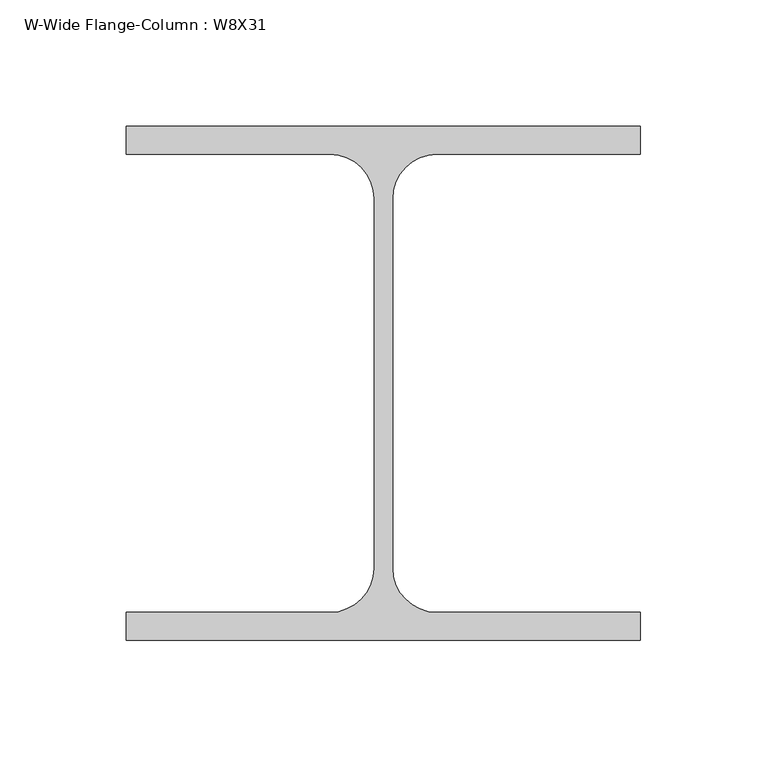
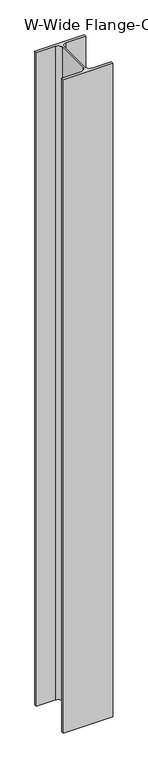
"""IFC4 building model written with IfcOpenShell, lengths in millimetres: column geometry, W-Wide Flange-Column : W8X31."""

from ifc_helpers import new_model, si_unit, point, frame_2d, origin, origin_with_axes, place, context, project, spatial, polyline, circle_curve, trimmed, segment, composite_curve, outline, extrude, source, transform, mapped, element, save


def w_wide_flange_column_w8x31_d6c08447(model_context):
    return source(origin(), model_context, "Body", "SweptSolid", [
        extrude(outline(composite_curve([segment(polyline([(101.6, 101.6), (101.6, 90.551), (21.1455, 90.551)]), True, "CONTINUOUS"), segment(trimmed(circle_curve(frame_2d((21.1455, 73.025)), 17.526), [point((21.1455, 90.551))], [point((3.6195, 73.025))], True, "CARTESIAN"), True, "CONTINUOUS"), segment(polyline([(3.6195, 73.025), (3.6195, -73.025)]), True, "CONTINUOUS"), segment(trimmed(circle_curve(frame_2d((21.1455, -73.025)), 17.526), [point((3.6195, -73.025))], [point((21.1455, -90.551))], True, "CARTESIAN"), True, "CONTINUOUS"), segment(polyline([(21.1455, -90.551), (101.6, -90.551), (101.6, -101.6), (-101.6, -101.6), (-101.6, -90.551), (-21.1455, -90.551)]), True, "CONTINUOUS"), segment(trimmed(circle_curve(frame_2d((-21.1455, -73.025)), 17.526), [point((-21.1455, -90.551))], [point((-3.6195, -73.025))], True, "CARTESIAN"), True, "CONTINUOUS"), segment(polyline([(-3.6195, -73.025), (-3.6195, 73.025)]), True, "CONTINUOUS"), segment(trimmed(circle_curve(frame_2d((-21.1455, 73.025)), 17.526), [point((-3.6195, 73.025))], [point((-21.1455, 90.551))], True, "CARTESIAN"), True, "CONTINUOUS"), segment(polyline([(-21.1455, 90.551), (-101.6, 90.551), (-101.6, 101.6), (101.6, 101.6)]), True, "CONTINUOUS")], self_intersect=False)), origin_with_axes(), (0.0, 0.0, 1.0), 2844.8),
    ])


if __name__ == "__main__":
    model = new_model("IFC4")
    model_context = context("Model", 3, world=origin())
    ifc_project = project(units=[si_unit("LENGTHUNIT", "METRE", prefix="MILLI")], contexts=[model_context])
    site = spatial("IfcSite", under=ifc_project)
    building = spatial("IfcBuilding", under=site)
    placement = place(None, origin())
    w_wide_flange_column_w8x31_shape = w_wide_flange_column_w8x31_d6c08447(model_context)
    element("IfcColumn", 1, ObjectType="W-Wide Flange-Column : W8X31", at=placement, inside=building, context=model_context, shape_type="MappedRepresentation", body=[
        mapped(w_wide_flange_column_w8x31_shape, transform((0.0, 0.0, 0.0), x_axis=(1.0, 0.0, 0.0), y_axis=(0.0, 1.0, 0.0), z_axis=(0.0, 0.0, 1.0))),
    ])
    save(model, "model.ifc")

# Revit data of these elements
# Type "W-Wide Flange-Column : W8X31"
#   Assembly Code = "B10"
#   W = 31
#   bf = 0' - 8"
#   d = 0' - 8"
#   k = 0' - 1 1/8"
#   kr = 0' - 0.69"
#   tf = 0' - 0.435"
#   tw = 0' - 0.285"
#   A = 0.0633333 SF
#   Structural Material [instance default] = Steel ASTM A992
# Element 1 (IfcColumn, "W-Wide Flange-Column : W8X31")
#   Materials on its faces: "Steel ASTM A992"
# Materials
#   "Steel ASTM A992": class "Metal", colour RGB 199 199 199, transparency 0, Description = "Structural steel 50ksi", Cost = 0
